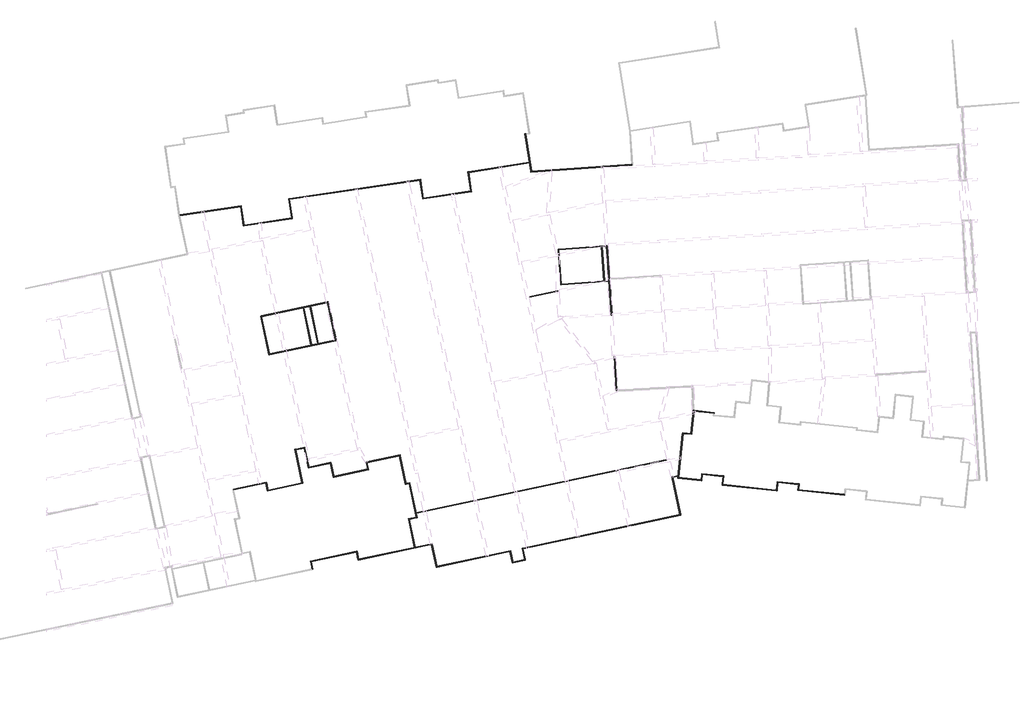
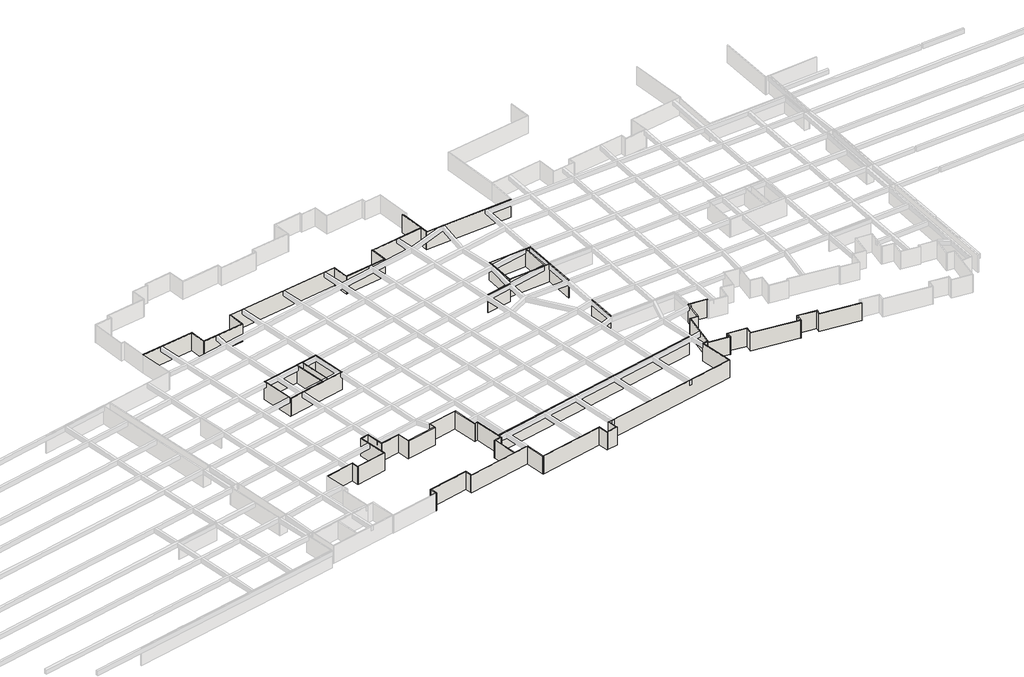
# One storey, part 3 of 14: 67 walls.
"""IFC4 building model written with IfcOpenShell, lengths in millimetres."""

from ifc_helpers import new_model, si_unit, origin, origin_with_axes, place, context, project, spatial, polyline, outline, extrude, faceted_brep, element, save

model = new_model("IFC4")

# Units and contexts
model_context = context("Model", 3, world=origin())
ifc_project = project(units=[si_unit("LENGTHUNIT", "METRE", prefix="MILLI")], contexts=[model_context])

# Site, building, storey
site = spatial("IfcSite", under=ifc_project)
building = spatial("IfcBuilding", under=site)
storey = spatial("IfcBuildingStorey", under=building, Name="户型图", Elevation=0.0)

# Walls
placement = place(None, origin())
element("IfcWall", 1, ObjectType="所有墙体", at=placement, inside=storey, context=model_context, shape_type="Brep", body=[
    faceted_brep([(-251184.7932427, -180181.6677158, 0.0), (-246225.4514721, -179127.5270809, 0.0), (-246108.07376, -179102.577678, 0.0), (-246108.07376, -179102.577678, 3300.0), (-246225.4514721, -179127.5270809, 3300.0), (-251184.7932427, -180181.6677158, 3300.0), (-251209.7426456, -180064.2900037, 0.0), (-251209.7426456, -180064.2900037, 3300.0), (-246133.0231629, -178985.1999659, 3300.0), (-246133.0231629, -178985.1999659, 0.0)], [[[0, 1, 2, 3, 4, 5]], [[6, 7, 8, 9]], [[2, 1, 0, 6, 9]], [[5, 4, 3, 8, 7]], [[0, 5, 7, 6]], [[3, 2, 9, 8]]]),
])
element("IfcWall", 2, ObjectType="所有墙体", at=placement, inside=storey, context=model_context, shape_type="Brep", body=[
    faceted_brep([(-246225.4514721, -179127.5270809, 0.0), (-245969.2063711, -180333.0654988, 0.0), (-245969.2063711, -180333.0654988, 3300.0), (-246225.4514721, -179127.5270809, 3300.0), (-246108.07376, -179102.577678, 0.0), (-246108.07376, -179102.577678, 3300.0), (-245876.7780619, -180190.7383838, 3300.0), (-245851.828659, -180308.1160959, 3300.0), (-245851.828659, -180308.1160959, 0.0), (-245876.7780619, -180190.7383838, 0.0)], [[[0, 1, 2, 3]], [[4, 5, 6, 7, 8, 9]], [[1, 0, 4, 9, 8]], [[3, 2, 7, 6, 5]], [[0, 3, 5, 4]], [[2, 1, 8, 7]]]),
])
element("IfcWall", 3, ObjectType="所有墙体", at=placement, inside=storey, context=model_context, shape_type="Brep", body=[
    faceted_brep([(-245851.828659, -180308.1160959, 0.0), (-240528.356814, -179176.5772244, 0.0), (-240528.356814, -179176.5772244, 3300.0), (-245851.828659, -180308.1160959, 3300.0), (-245876.7780619, -180190.7383838, 0.0), (-245876.7780619, -180190.7383838, 3300.0), (-240670.683929, -179084.1489152, 3300.0), (-240553.3062169, -179059.1995123, 3300.0), (-240553.3062169, -179059.1995123, 0.0), (-240670.683929, -179084.1489152, 0.0)], [[[0, 1, 2, 3]], [[4, 5, 6, 7, 8, 9]], [[1, 0, 4, 9, 8]], [[3, 2, 7, 6, 5]], [[0, 3, 5, 4]], [[2, 1, 8, 7]]]),
])
element("IfcWall", 4, ObjectType="所有墙体", at=placement, inside=storey, context=model_context, shape_type="Brep", body=[
    faceted_brep([(-240553.3062169, -179059.1995123, 0.0), (-241623.2362036, -174025.5746821, 0.0), (-241648.1856065, -173908.19697, 0.0), (-241648.1856065, -173908.19697, 3300.0), (-241623.2362036, -174025.5746821, 3300.0), (-240553.3062169, -179059.1995123, 3300.0), (-240670.683929, -179084.1489152, 0.0), (-240670.683929, -179084.1489152, 3300.0), (-241765.5633186, -173933.1463729, 3300.0), (-241765.5633186, -173933.1463729, 0.0)], [[[0, 1, 2, 3, 4, 5]], [[6, 7, 8, 9]], [[2, 1, 0, 6, 9]], [[5, 4, 3, 8, 7]], [[0, 5, 7, 6]], [[3, 2, 9, 8]]]),
])
element("IfcWall", 5, ObjectType="所有墙体", at=placement, inside=storey, context=model_context, shape_type="Brep", body=[
    faceted_brep([(-241623.2362036, -174025.5746821, 0.0), (-240338.9777317, -173752.597117, 0.0), (-240221.6000196, -173727.6477141, 0.0), (-240221.6000196, -173727.6477141, 3300.0), (-240338.9777317, -173752.597117, 3300.0), (-241623.2362036, -174025.5746821, 3300.0), (-241648.1856065, -173908.19697, 0.0), (-241648.1856065, -173908.19697, 3300.0), (-240246.5494225, -173610.270002, 3300.0), (-240246.5494225, -173610.270002, 0.0)], [[[0, 1, 2, 3, 4, 5]], [[6, 7, 8, 9]], [[2, 1, 0, 6, 9]], [[5, 4, 3, 8, 7]], [[0, 5, 7, 6]], [[3, 2, 9, 8]]]),
])
element("IfcWall", 6, ObjectType="所有墙体", at=placement, inside=storey, context=model_context, shape_type="Brep", body=[
    faceted_brep([(-240338.9777317, -173752.597117, 0.0), (-239692.5763399, -176793.6765678, 0.0), (-239692.5763399, -176793.6765678, 3300.0), (-240338.9777317, -173752.597117, 3300.0), (-240221.6000196, -173727.6477141, 0.0), (-240221.6000196, -173727.6477141, 3300.0), (-239600.1480307, -176651.3494528, 3300.0), (-239575.1986278, -176768.7271649, 3300.0), (-239575.1986278, -176768.7271649, 0.0), (-239600.1480307, -176651.3494528, 0.0)], [[[0, 1, 2, 3]], [[4, 5, 6, 7, 8, 9]], [[1, 0, 4, 9, 8]], [[3, 2, 7, 6, 5]], [[0, 3, 5, 4]], [[2, 1, 8, 7]]]),
])
element("IfcWall", 7, ObjectType="所有墙体", at=placement, inside=storey, context=model_context, shape_type="Brep", body=[
    faceted_brep([(-239575.1986278, -176768.7271649, 0.0), (-236288.0048587, -176070.0125598, 0.0), (-236170.6271466, -176045.0631569, 0.0), (-236170.6271466, -176045.0631569, 3300.0), (-236288.0048587, -176070.0125598, 3300.0), (-239575.1986278, -176768.7271649, 3300.0), (-239600.1480307, -176651.3494528, 0.0), (-239600.1480307, -176651.3494528, 3300.0), (-236195.5765495, -175927.6854448, 3300.0), (-236195.5765495, -175927.6854448, 0.0)], [[[0, 1, 2, 3, 4, 5]], [[6, 7, 8, 9]], [[2, 1, 0, 6, 9]], [[5, 4, 3, 8, 7]], [[0, 5, 7, 6]], [[3, 2, 9, 8]]]),
])
element("IfcWall", 8, ObjectType="所有墙体", at=placement, inside=storey, context=model_context, shape_type="Brep", body=[
    faceted_brep([(-236288.0048587, -176070.0125598, 0.0), (-235830.5991389, -178221.9372814, 0.0), (-235830.5991389, -178221.9372814, 3300.0), (-236288.0048587, -176070.0125598, 3300.0), (-236170.6271466, -176045.0631569, 0.0), (-236170.6271466, -176045.0631569, 3300.0), (-235738.1708297, -178079.6101664, 3300.0), (-235713.2214268, -178196.9878785, 3300.0), (-235713.2214268, -178196.9878785, 0.0), (-235738.1708297, -178079.6101664, 0.0)], [[[0, 1, 2, 3]], [[4, 5, 6, 7, 8, 9]], [[1, 0, 4, 9, 8]], [[3, 2, 7, 6, 5]], [[0, 3, 5, 4]], [[2, 1, 8, 7]]]),
])
element("IfcWall", 9, ObjectType="所有墙体", at=placement, inside=storey, context=model_context, shape_type="Brep", body=[
    faceted_brep([(-235713.2214268, -178196.9878785, 0.0), (-230395.6661839, -177066.7066196, 0.0), (-230395.6661839, -177066.7066196, 3300.0), (-235713.2214268, -178196.9878785, 3300.0), (-235738.1708297, -178079.6101664, 0.0), (-235738.1708297, -178079.6101664, 3300.0), (-230537.9932989, -176974.2783104, 3300.0), (-230420.6155868, -176949.3289075, 3300.0), (-230420.6155868, -176949.3289075, 0.0), (-230537.9932989, -176974.2783104, 0.0)], [[[0, 1, 2, 3]], [[4, 5, 6, 7, 8, 9]], [[1, 0, 4, 9, 8]], [[3, 2, 7, 6, 5]], [[0, 3, 5, 4]], [[2, 1, 8, 7]]]),
])
element("IfcWall", 10, ObjectType="所有墙体", at=placement, inside=storey, context=model_context, shape_type="Brep", body=[
    faceted_brep([(-230420.6155868, -176949.3289075, 0.0), (-230627.4632891, -175976.186979, 0.0), (-230652.412692, -175858.809267, 0.0), (-230652.412692, -175858.809267, 3300.0), (-230627.4632891, -175976.186979, 3300.0), (-230420.6155868, -176949.3289075, 3300.0), (-230537.9932989, -176974.2783104, 0.0), (-230537.9932989, -176974.2783104, 3300.0), (-230769.7904041, -175883.7586699, 3300.0), (-230769.7904041, -175883.7586699, 0.0)], [[[0, 1, 2, 3, 4, 5]], [[6, 7, 8, 9]], [[2, 1, 0, 6, 9]], [[5, 4, 3, 8, 7]], [[0, 5, 7, 6]], [[3, 2, 9, 8]]]),
])
element("IfcWall", 11, ObjectType="所有墙体", at=placement, inside=storey, context=model_context, shape_type="Brep", body=[
    faceted_brep([(-230627.4632891, -175976.186979, 0.0), (-225651.5563884, -174918.525317, 0.0), (-225534.1786764, -174893.5759141, 0.0), (-225534.1786764, -174893.5759141, 3300.0), (-225651.5563884, -174918.525317, 3300.0), (-230627.4632891, -175976.186979, 3300.0), (-230652.412692, -175858.809267, 0.0), (-230652.412692, -175858.809267, 3300.0), (-225559.1280793, -174776.1982021, 3300.0), (-225559.1280793, -174776.1982021, 0.0)], [[[0, 1, 2, 3, 4, 5]], [[6, 7, 8, 9]], [[2, 1, 0, 6, 9]], [[5, 4, 3, 8, 7]], [[0, 5, 7, 6]], [[3, 2, 9, 8]]]),
])
element("IfcWall", 12, ObjectType="所有墙体", at=placement, inside=storey, context=model_context, shape_type="Brep", body=[
    faceted_brep([(-225651.5563884, -174918.525317, 0.0), (-224715.2696958, -179323.4078824, 0.0), (-224715.2696958, -179323.4078824, 3300.0), (-225651.5563884, -174918.525317, 3300.0), (-225534.1786764, -174893.5759141, 0.0), (-225534.1786764, -174893.5759141, 3300.0), (-224622.8413866, -179181.0807674, 3300.0), (-224597.8919837, -179298.4584795, 3300.0), (-224597.8919837, -179298.4584795, 0.0), (-224622.8413866, -179181.0807674, 0.0)], [[[0, 1, 2, 3]], [[4, 5, 6, 7, 8, 9]], [[1, 0, 4, 9, 8]], [[3, 2, 7, 6, 5]], [[0, 3, 5, 4]], [[2, 1, 8, 7]]]),
])
element("IfcWall", 13, ObjectType="所有墙体", at=placement, inside=storey, context=model_context, shape_type="Brep", body=[
    faceted_brep([(-224597.8919837, -179298.4584795, 0.0), (-224155.9078939, -179204.5118611, 0.0), (-224038.5301818, -179179.5624582, 0.0), (-224038.5301818, -179179.5624582, 3300.0), (-224155.9078939, -179204.5118611, 3300.0), (-224597.8919837, -179298.4584795, 3300.0), (-224622.8413866, -179181.0807674, 0.0), (-224622.8413866, -179181.0807674, 3300.0), (-224063.4795847, -179062.1847461, 3300.0), (-224063.4795847, -179062.1847461, 0.0)], [[[0, 1, 2, 3, 4, 5]], [[6, 7, 8, 9]], [[2, 1, 0, 6, 9]], [[5, 4, 3, 8, 7]], [[0, 5, 7, 6]], [[3, 2, 9, 8]]]),
])
element("IfcWall", 14, ObjectType="所有墙体", at=placement, inside=storey, context=model_context, shape_type="Brep", body=[
    faceted_brep([(-224155.9078939, -179204.5118611, 0.0), (-223057.3689575, -184372.7312177, 0.0), (-223032.4195546, -184490.1089298, 0.0), (-223032.4195546, -184490.1089298, 3300.0), (-223057.3689575, -184372.7312177, 3300.0), (-224155.9078939, -179204.5118611, 3300.0), (-224038.5301818, -179179.5624582, 0.0), (-224038.5301818, -179179.5624582, 3300.0), (-223083.6040764, -183672.1365659, 3300.0), (-223058.6546735, -183789.5142779, 3300.0), (-222915.0418425, -184465.1595269, 3300.0), (-222915.0418425, -184465.1595269, 0.0), (-223058.6546735, -183789.5142779, 0.0), (-223083.6040764, -183672.1365659, 0.0)], [[[0, 1, 2, 3, 4, 5]], [[6, 7, 8, 9, 10, 11, 12, 13]], [[2, 1, 0, 6, 13, 12, 11]], [[5, 4, 3, 10, 9, 8, 7]], [[0, 5, 7, 6]], [[3, 2, 11, 10]]]),
])
element("IfcWall", 15, ObjectType="所有墙体", at=placement, inside=storey, context=model_context, shape_type="Brep", body=[
    faceted_brep([(-223057.3689575, -184372.7312177, 0.0), (-224264.2132514, -184629.2538913, 0.0), (-224264.2132514, -184629.2538913, 3300.0), (-223057.3689575, -184372.7312177, 3300.0), (-223032.4195546, -184490.1089298, 0.0), (-223032.4195546, -184490.1089298, 3300.0), (-224121.8861364, -184721.6822004, 3300.0), (-224239.2638485, -184746.6316033, 3300.0), (-224239.2638485, -184746.6316033, 0.0), (-224121.8861364, -184721.6822004, 0.0)], [[[0, 1, 2, 3]], [[4, 5, 6, 7, 8, 9]], [[1, 0, 4, 9, 8]], [[3, 2, 7, 6, 5]], [[0, 3, 5, 4]], [[2, 1, 8, 7]]]),
])
element("IfcWall", 16, ObjectType="所有墙体", at=placement, inside=storey, context=model_context, shape_type="SweptSolid", body=[
    extrude(outline(polyline([(-223330.1960749, -189023.4592223), (-224239.2638485, -184746.6316033), (-224121.8861364, -184721.6822004), (-223212.8183628, -188998.5098194), (-223330.1960749, -189023.4592223)])), origin_with_axes(), (0.0, 0.0, 1.0), 3300.0),
])
element("IfcWall", 17, ObjectType="所有墙体", at=placement, inside=storey, context=model_context, shape_type="Brep", body=[
    faceted_brep([(-220629.7896191, -188449.4701109, 0.0), (-223212.8183628, -188998.5098194, 0.0), (-223330.1960749, -189023.4592223, 0.0), (-231918.3320094, -190848.9238676, 0.0), (-232035.7097215, -190873.8732705, 0.0), (-232035.7097215, -190873.8732705, 3300.0), (-231918.3320094, -190848.9238676, 3300.0), (-223330.1960749, -189023.4592223, 3300.0), (-223212.8183628, -188998.5098194, 3300.0), (-220629.7896191, -188449.4701109, 3300.0), (-220604.8402162, -188566.847823, 0.0), (-220604.8402162, -188566.847823, 3300.0), (-220722.2179283, -188591.7972259, 3300.0), (-232010.7603186, -190991.2509826, 3300.0), (-232010.7603186, -190991.2509826, 0.0), (-220722.2179283, -188591.7972259, 0.0)], [[[0, 1, 2, 3, 4, 5, 6, 7, 8, 9]], [[10, 11, 12, 13, 14, 15]], [[4, 3, 2, 1, 0, 10, 15, 14]], [[9, 8, 7, 6, 5, 13, 12, 11]], [[5, 4, 14, 13]], [[0, 9, 11, 10]]]),
])
element("IfcWall", 18, ObjectType="所有墙体", at=placement, inside=storey, context=model_context, shape_type="Brep", body=[
    faceted_brep([(-231918.3320094, -190848.9238676, 0.0), (-232179.3992418, -189620.6991054, 0.0), (-232179.3992418, -189620.6991054, 3300.0), (-231918.3320094, -190848.9238676, 3300.0), (-232035.7097215, -190873.8732705, 0.0), (-232035.7097215, -190873.8732705, 3300.0), (-232271.827551, -189763.0262204, 3300.0), (-232296.7769539, -189645.6485083, 3300.0), (-232296.7769539, -189645.6485083, 0.0), (-232271.827551, -189763.0262204, 0.0)], [[[0, 1, 2, 3]], [[4, 5, 6, 7, 8, 9]], [[1, 0, 4, 9, 8]], [[3, 2, 7, 6, 5]], [[0, 3, 5, 4]], [[2, 1, 8, 7]]]),
])
element("IfcWall", 19, ObjectType="所有墙体", at=placement, inside=storey, context=model_context, shape_type="Brep", body=[
    faceted_brep([(-232296.7769539, -189645.6485083, 0.0), (-239359.5403512, -191146.885212, 0.0), (-239359.5403512, -191146.885212, 3300.0), (-232296.7769539, -189645.6485083, 3300.0), (-232271.827551, -189763.0262204, 0.0), (-232271.827551, -189763.0262204, 3300.0), (-239217.2132362, -191239.3135211, 3300.0), (-239334.5909483, -191264.262924, 3300.0), (-239334.5909483, -191264.262924, 0.0), (-239217.2132362, -191239.3135211, 0.0)], [[[0, 1, 2, 3]], [[4, 5, 6, 7, 8, 9]], [[1, 0, 4, 9, 8]], [[3, 2, 7, 6, 5]], [[0, 3, 5, 4]], [[2, 1, 8, 7]]]),
])
element("IfcWall", 20, ObjectType="所有墙体", at=placement, inside=storey, context=model_context, shape_type="Brep", body=[
    faceted_brep([(-239334.5909483, -191264.262924, 0.0), (-239110.0463222, -192320.6623328, 0.0), (-239085.0969193, -192438.0400449, 0.0), (-239085.0969193, -192438.0400449, 3300.0), (-239110.0463222, -192320.6623328, 3300.0), (-239334.5909483, -191264.262924, 3300.0), (-239217.2132362, -191239.3135211, 0.0), (-239217.2132362, -191239.3135211, 3300.0), (-238967.7192072, -192413.090642, 3300.0), (-238967.7192072, -192413.090642, 0.0)], [[[0, 1, 2, 3, 4, 5]], [[6, 7, 8, 9]], [[2, 1, 0, 6, 9]], [[5, 4, 3, 8, 7]], [[0, 5, 7, 6]], [[3, 2, 9, 8]]]),
])
element("IfcWall", 21, ObjectType="所有墙体", at=placement, inside=storey, context=model_context, shape_type="Brep", body=[
    faceted_brep([(-182065.556888, -171503.9612716, 0.0), (-181945.9953144, -171514.4215539, 0.0), (-180665.2470066, -171626.4725117, 0.0), (-180665.2470066, -171626.4725117, 3300.0), (-181945.9953144, -171514.4215539, 3300.0), (-182065.556888, -171503.9612716, 3300.0), (-182053.0115616, -171384.6004649, 0.0), (-182053.0115616, -171384.6004649, 3300.0), (-180772.2632539, -171496.6514227, 3300.0), (-180652.7016803, -171507.111705, 3300.0), (-180652.7016803, -171507.111705, 0.0), (-180772.2632539, -171496.6514227, 0.0)], [[[0, 1, 2, 3, 4, 5]], [[6, 7, 8, 9, 10, 11]], [[2, 1, 0, 6, 11, 10]], [[5, 4, 3, 9, 8, 7]], [[3, 2, 10, 9]], [[0, 5, 7, 6]]]),
])
element("IfcWall", 22, ObjectType="所有墙体", at=placement, inside=storey, context=model_context, shape_type="Brep", body=[
    faceted_brep([(-180652.7016803, -171507.111705, 0.0), (-180289.0530565, -168047.2261654, 0.0), (-180276.5096409, -167927.8835379, 0.0), (-180276.5096409, -167927.8835379, 3300.0), (-180289.0530565, -168047.2261654, 3300.0), (-180652.7016803, -171507.111705, 3300.0), (-180772.2632539, -171496.6514227, 0.0), (-180772.2632539, -171496.6514227, 3300.0), (-180402.6175703, -167979.7076703, 3300.0), (-180395.8522684, -167915.3401223, 3300.0), (-180395.8522684, -167915.3401223, 0.0), (-180402.6175703, -167979.7076703, 0.0), (-180285.2168381, -167926.9683746, 0.0), (-180285.2168381, -167926.9683746, 3300.0)], [[[0, 1, 2, 3, 4, 5]], [[6, 7, 8, 9, 10, 11]], [[2, 1, 0, 6, 11, 10, 12]], [[5, 4, 3, 13, 9, 8, 7]], [[0, 5, 7, 6]], [[3, 2, 12, 10, 9, 13]]]),
])
element("IfcWall", 23, ObjectType="所有墙体", at=placement, inside=storey, context=model_context, shape_type="Brep", body=[
    faceted_brep([(-180289.0530565, -168047.2261654, 0.0), (-177282.9502682, -168363.1803001, 0.0), (-177163.6076407, -168375.7237157, 0.0), (-177163.6076407, -168375.7237157, 3300.0), (-177282.9502682, -168363.1803001, 3300.0), (-180289.0530565, -168047.2261654, 3300.0), (-180276.5096409, -167927.8835379, 0.0), (-180276.5096409, -167927.8835379, 3300.0), (-177151.0642251, -168256.3810882, 3300.0), (-177151.0642251, -168256.3810882, 0.0)], [[[0, 1, 2, 3, 4, 5]], [[6, 7, 8, 9]], [[2, 1, 0, 6, 9]], [[5, 4, 3, 8, 7]], [[0, 5, 7, 6]], [[3, 2, 9, 8]]]),
])
element("IfcWall", 24, ObjectType="所有墙体", at=placement, inside=storey, context=model_context, shape_type="Brep", body=[
    faceted_brep([(-157110.1034337, -180872.9468522, 0.0), (-164149.4886008, -180133.0776575, 0.0), (-164268.8312282, -180120.5342419, 0.0), (-164268.8312282, -180120.5342419, 3300.0), (-164149.4886008, -180133.0776575, 3300.0), (-157110.1034337, -180872.9468522, 3300.0), (-157122.6468493, -180992.2894796, 0.0), (-157122.6468493, -180992.2894796, 3300.0), (-164281.3746438, -180239.8768693, 3300.0), (-164281.3746438, -180239.8768693, 0.0)], [[[0, 1, 2, 3, 4, 5]], [[6, 7, 8, 9]], [[2, 1, 0, 6, 9]], [[5, 4, 3, 8, 7]], [[0, 5, 7, 6]], [[3, 2, 9, 8]]]),
])
element("IfcWall", 25, ObjectType="所有墙体", at=placement, inside=storey, context=model_context, shape_type="Brep", body=[
    faceted_brep([(-164149.4886008, -180133.0776575, 0.0), (-164056.3781259, -179247.1906647, 0.0), (-164056.3781259, -179247.1906647, 3300.0), (-164149.4886008, -180133.0776575, 3300.0), (-164268.8312282, -180120.5342419, 0.0), (-164268.8312282, -180120.5342419, 3300.0), (-164188.2641689, -179353.9898766, 3300.0), (-164175.7207533, -179234.6472492, 3300.0), (-164175.7207533, -179234.6472492, 0.0), (-164188.2641689, -179353.9898766, 0.0)], [[[0, 1, 2, 3]], [[4, 5, 6, 7, 8, 9]], [[1, 0, 4, 9, 8]], [[3, 2, 7, 6, 5]], [[0, 3, 5, 4]], [[2, 1, 8, 7]]]),
])
element("IfcWall", 26, ObjectType="所有墙体", at=placement, inside=storey, context=model_context, shape_type="Brep", body=[
    faceted_brep([(-164175.7207533, -179234.6472492, 0.0), (-167459.4955166, -178889.5086139, 0.0), (-167459.4955166, -178889.5086139, 3300.0), (-164175.7207533, -179234.6472492, 3300.0), (-164188.2641689, -179353.9898766, 0.0), (-164188.2641689, -179353.9898766, 3300.0), (-167352.6963048, -179021.3946569, 3300.0), (-167472.0389322, -179008.8512413, 3300.0), (-167472.0389322, -179008.8512413, 0.0), (-167352.6963048, -179021.3946569, 0.0)], [[[0, 1, 2, 3]], [[4, 5, 6, 7, 8, 9]], [[1, 0, 4, 9, 8]], [[3, 2, 7, 6, 5]], [[0, 3, 5, 4]], [[2, 1, 8, 7]]]),
])
element("IfcWall", 27, ObjectType="所有墙体", at=placement, inside=storey, context=model_context, shape_type="Brep", body=[
    faceted_brep([(-167472.0389322, -179008.8512413, 0.0), (-167597.4730882, -180202.2775158, 0.0), (-167610.0165037, -180321.6201432, 0.0), (-167610.0165037, -180321.6201432, 3300.0), (-167597.4730882, -180202.2775158, 3300.0), (-167472.0389322, -179008.8512413, 3300.0), (-167352.6963048, -179021.3946569, 0.0), (-167352.6963048, -179021.3946569, 3300.0), (-167490.6738763, -180334.1635588, 3300.0), (-167490.6738763, -180334.1635588, 0.0)], [[[0, 1, 2, 3, 4, 5]], [[6, 7, 8, 9]], [[2, 1, 0, 6, 9]], [[5, 4, 3, 8, 7]], [[0, 5, 7, 6]], [[3, 2, 9, 8]]]),
])
element("IfcWall", 28, ObjectType="所有墙体", at=placement, inside=storey, context=model_context, shape_type="Brep", body=[
    faceted_brep([(-167597.4730882, -180202.2775158, 0.0), (-175829.3978828, -179337.0673554, 0.0), (-175948.7405103, -179324.5239399, 0.0), (-175948.7405103, -179324.5239399, 3300.0), (-175829.3978828, -179337.0673554, 3300.0), (-167597.4730882, -180202.2775158, 3300.0), (-167610.0165037, -180321.6201432, 0.0), (-167610.0165037, -180321.6201432, 3300.0), (-175961.2839258, -179443.8665673, 3300.0), (-175961.2839258, -179443.8665673, 0.0)], [[[0, 1, 2, 3, 4, 5]], [[6, 7, 8, 9]], [[2, 1, 0, 6, 9]], [[5, 4, 3, 8, 7]], [[0, 5, 7, 6]], [[3, 2, 9, 8]]]),
])
element("IfcWall", 29, ObjectType="所有墙体", at=placement, inside=storey, context=model_context, shape_type="Brep", body=[
    faceted_brep([(-175829.3978828, -179337.0673554, 0.0), (-175691.4203113, -178024.2984536, 0.0), (-175691.4203113, -178024.2984536, 3300.0), (-175829.3978828, -179337.0673554, 3300.0), (-175948.7405103, -179324.5239399, 0.0), (-175948.7405103, -179324.5239399, 3300.0), (-175823.3063543, -178131.0976654, 3300.0), (-175810.7629387, -178011.755038, 3300.0), (-175810.7629387, -178011.755038, 0.0), (-175823.3063543, -178131.0976654, 0.0)], [[[0, 1, 2, 3]], [[4, 5, 6, 7, 8, 9]], [[1, 0, 4, 9, 8]], [[3, 2, 7, 6, 5]], [[0, 3, 5, 4]], [[2, 1, 8, 7]]]),
])
element("IfcWall", 30, ObjectType="所有墙体", at=placement, inside=storey, context=model_context, shape_type="Brep", body=[
    faceted_brep([(-175810.7629387, -178011.755038, 0.0), (-179092.6851935, -177666.8111092, 0.0), (-179092.6851935, -177666.8111092, 3300.0), (-175810.7629387, -178011.755038, 3300.0), (-175823.3063543, -178131.0976654, 0.0), (-175823.3063543, -178131.0976654, 3300.0), (-178985.8859816, -177798.6971522, 3300.0), (-179105.228609, -177786.1537366, 3300.0), (-179105.228609, -177786.1537366, 0.0), (-178985.8859816, -177798.6971522, 0.0)], [[[0, 1, 2, 3]], [[4, 5, 6, 7, 8, 9]], [[1, 0, 4, 9, 8]], [[3, 2, 7, 6, 5]], [[0, 3, 5, 4]], [[2, 1, 8, 7]]]),
])
element("IfcWall", 31, ObjectType="所有墙体", at=placement, inside=storey, context=model_context, shape_type="Brep", body=[
    faceted_brep([(-179105.228609, -177786.1537366, 0.0), (-179192.313451, -178614.7106614, 0.0), (-179204.8568666, -178734.0532889, 0.0), (-179204.8568666, -178734.0532889, 3300.0), (-179192.313451, -178614.7106614, 3300.0), (-179105.228609, -177786.1537366, 3300.0), (-178985.8859816, -177798.6971522, 0.0), (-178985.8859816, -177798.6971522, 3300.0), (-179085.5142391, -178746.5967045, 3300.0), (-179085.5142391, -178746.5967045, 0.0)], [[[0, 1, 2, 3, 4, 5]], [[6, 7, 8, 9]], [[2, 1, 0, 6, 9]], [[5, 4, 3, 8, 7]], [[0, 5, 7, 6]], [[3, 2, 9, 8]]]),
])
element("IfcWall", 32, ObjectType="所有墙体", at=placement, inside=storey, context=model_context, shape_type="Brep", body=[
    faceted_brep([(-179192.313451, -178614.7106614, 0.0), (-182654.0245934, -178250.8701591, 0.0), (-182773.3672209, -178238.3267435, 0.0), (-182773.3672209, -178238.3267435, 3300.0), (-182654.0245934, -178250.8701591, 3300.0), (-179192.313451, -178614.7106614, 3300.0), (-179204.8568666, -178734.0532889, 0.0), (-179204.8568666, -178734.0532889, 3300.0), (-182785.9106365, -178357.669371, 3300.0), (-182785.9106365, -178357.669371, 0.0)], [[[0, 1, 2, 3, 4, 5]], [[6, 7, 8, 9]], [[2, 1, 0, 6, 9]], [[5, 4, 3, 8, 7]], [[0, 5, 7, 6]], [[3, 2, 9, 8]]]),
])
element("IfcWall", 33, ObjectType="所有墙体", at=placement, inside=storey, context=model_context, shape_type="Brep", body=[
    faceted_brep([(-182654.0245934, -178250.8701591, 0.0), (-181945.9953144, -171514.4215539, 0.0), (-181945.9953144, -171514.4215539, 3300.0), (-182654.0245934, -178250.8701591, 3300.0), (-182773.3672209, -178238.3267435, 0.0), (-182773.3672209, -178238.3267435, 3300.0), (-182757.9194792, -178091.3512993, 3300.0), (-182744.7305516, -177965.8670348, 3300.0), (-182065.556888, -171503.9612716, 3300.0), (-182065.556888, -171503.9612716, 0.0), (-182744.7305516, -177965.8670348, 0.0), (-182757.9194792, -178091.3512993, 0.0)], [[[0, 1, 2, 3]], [[4, 5, 6, 7, 8, 9, 10, 11]], [[1, 0, 4, 11, 10, 9]], [[3, 2, 8, 7, 6, 5]], [[2, 1, 9, 8]], [[0, 3, 5, 4]]]),
])
element("IfcWall", 34, ObjectType="所有墙体", at=placement, inside=storey, context=model_context, shape_type="Brep", body=[
    faceted_brep([(-205290.7605884, -131109.081479, 0.0), (-206189.3856367, -125435.3862189, 0.0), (-206208.1577725, -125316.863618, 0.0), (-206208.1577725, -125316.863618, 3300.0), (-206189.3856367, -125435.3862189, 3300.0), (-205290.7605884, -131109.081479, 3300.0), (-205410.9255383, -131117.4842309, 0.0), (-205410.9255383, -131117.4842309, 3300.0), (-205617.1977326, -129815.132852, 3300.0), (-205635.9698684, -129696.6102511, 3300.0), (-206326.6803734, -125335.6357538, 3300.0), (-206326.6803734, -125335.6357538, 0.0), (-205635.9698684, -129696.6102511, 0.0), (-205617.1977326, -129815.132852, 0.0)], [[[0, 1, 2, 3, 4, 5]], [[6, 7, 8, 9, 10, 11, 12, 13]], [[2, 1, 0, 6, 13, 12, 11]], [[5, 4, 3, 10, 9, 8, 7]], [[3, 2, 11, 10]], [[0, 5, 7, 6]]]),
])
element("IfcWall", 35, ObjectType="所有墙体", at=placement, inside=storey, context=model_context, shape_type="Brep", body=[
    faceted_brep([(-259497.8296146, -137947.3843831, 0.0), (-259493.9278671, -137946.8113411, 0.0), (-250107.6507443, -136568.2671346, 0.0), (-249988.9243897, -136550.8300265, 0.0), (-249988.9243897, -136550.8300265, 3300.0), (-250107.6507443, -136568.2671346, 3300.0), (-259493.9278671, -137946.8113411, 3300.0), (-259497.8296146, -137947.3843831, 3300.0), (-259515.2667226, -137828.6580286, 0.0), (-259515.2667226, -137828.6580286, 3300.0), (-250006.3614978, -136432.103672, 3300.0), (-250006.3614978, -136432.103672, 0.0)], [[[0, 1, 2, 3, 4, 5, 6, 7]], [[8, 9, 10, 11]], [[3, 2, 1, 0, 8, 11]], [[7, 6, 5, 4, 10, 9]], [[0, 7, 9, 8]], [[4, 3, 11, 10]]]),
])
element("IfcWall", 36, ObjectType="所有墙体", at=placement, inside=storey, context=model_context, shape_type="Brep", body=[
    faceted_brep([(-250107.6507443, -136568.2671346, 0.0), (-249675.1126294, -139513.3468741, 0.0), (-249675.1126294, -139513.3468741, 3300.0), (-250107.6507443, -136568.2671346, 3300.0), (-249988.9243897, -136550.8300265, 0.0), (-249988.9243897, -136550.8300265, 3300.0), (-249573.8233829, -139377.1834115, 3300.0), (-249556.3862748, -139495.9097661, 3300.0), (-249556.3862748, -139495.9097661, 0.0), (-249573.8233829, -139377.1834115, 0.0)], [[[0, 1, 2, 3]], [[4, 5, 6, 7, 8, 9]], [[1, 0, 4, 9, 8]], [[3, 2, 7, 6, 5]], [[0, 3, 5, 4]], [[2, 1, 8, 7]]]),
])
element("IfcWall", 37, ObjectType="所有墙体", at=placement, inside=storey, context=model_context, shape_type="Brep", body=[
    faceted_brep([(-249556.3862748, -139495.9097661, 0.0), (-242128.8165149, -138405.0370881, 0.0), (-242128.8165149, -138405.0370881, 3300.0), (-249556.3862748, -139495.9097661, 3300.0), (-249573.8233829, -139377.1834115, 0.0), (-249573.8233829, -139377.1834115, 3300.0), (-242264.9799775, -138303.7478416, 3300.0), (-242146.253623, -138286.3107336, 3300.0), (-242146.253623, -138286.3107336, 0.0), (-242264.9799775, -138303.7478416, 0.0)], [[[0, 1, 2, 3]], [[4, 5, 6, 7, 8, 9]], [[1, 0, 4, 9, 8]], [[3, 2, 7, 6, 5]], [[0, 3, 5, 4]], [[2, 1, 8, 7]]]),
])
element("IfcWall", 38, ObjectType="所有墙体", at=placement, inside=storey, context=model_context, shape_type="Brep", body=[
    faceted_brep([(-242146.253623, -138286.3107336, 0.0), (-242564.7442158, -135436.8782245, 0.0), (-242582.1813238, -135318.15187, 0.0), (-242582.1813238, -135318.15187, 3300.0), (-242564.7442158, -135436.8782245, 3300.0), (-242146.253623, -138286.3107336, 3300.0), (-242264.9799775, -138303.7478416, 0.0), (-242264.9799775, -138303.7478416, 3300.0), (-242700.9076783, -135335.588978, 3300.0), (-242700.9076783, -135335.588978, 0.0)], [[[0, 1, 2, 3, 4, 5]], [[6, 7, 8, 9]], [[2, 1, 0, 6, 9]], [[5, 4, 3, 8, 7]], [[0, 5, 7, 6]], [[3, 2, 9, 8]]]),
])
element("IfcWall", 39, ObjectType="所有墙体", at=placement, inside=storey, context=model_context, shape_type="Brep", body=[
    faceted_brep([(-242564.7442158, -135436.8782245, 0.0), (-222499.9902977, -132490.006967, 0.0), (-222381.2639432, -132472.5698589, 0.0), (-222381.2639432, -132472.5698589, 3300.0), (-222499.9902977, -132490.006967, 3300.0), (-242564.7442158, -135436.8782245, 3300.0), (-242582.1813238, -135318.15187, 0.0), (-242582.1813238, -135318.15187, 3300.0), (-222398.7010512, -132353.8435044, 3300.0), (-222398.7010512, -132353.8435044, 0.0)], [[[0, 1, 2, 3, 4, 5]], [[6, 7, 8, 9]], [[2, 1, 0, 6, 9]], [[5, 4, 3, 8, 7]], [[0, 5, 7, 6]], [[3, 2, 9, 8]]]),
])
element("IfcWall", 40, ObjectType="所有墙体", at=placement, inside=storey, context=model_context, shape_type="Brep", body=[
    faceted_brep([(-222499.9902977, -132490.006967, 0.0), (-222078.5935203, -135359.2272018, 0.0), (-222078.5935203, -135359.2272018, 3300.0), (-222499.9902977, -132490.006967, 3300.0), (-222381.2639432, -132472.5698589, 0.0), (-222381.2639432, -132472.5698589, 3300.0), (-221977.3042738, -135223.0637392, 3300.0), (-221959.8671657, -135341.7900938, 3300.0), (-221959.8671657, -135341.7900938, 0.0), (-221977.3042738, -135223.0637392, 0.0)], [[[0, 1, 2, 3]], [[4, 5, 6, 7, 8, 9]], [[1, 0, 4, 9, 8]], [[3, 2, 7, 6, 5]], [[0, 3, 5, 4]], [[2, 1, 8, 7]]]),
])
element("IfcWall", 41, ObjectType="所有墙体", at=placement, inside=storey, context=model_context, shape_type="Brep", body=[
    faceted_brep([(-221959.8671657, -135341.7900938, 0.0), (-214539.6288625, -134251.9941726, 0.0), (-214539.6288625, -134251.9941726, 3300.0), (-221959.8671657, -135341.7900938, 3300.0), (-221977.3042738, -135223.0637392, 0.0), (-221977.3042738, -135223.0637392, 3300.0), (-214675.7923251, -134150.7049261, 3300.0), (-214557.0659706, -134133.267818, 3300.0), (-214557.0659706, -134133.267818, 0.0), (-214675.7923251, -134150.7049261, 0.0)], [[[0, 1, 2, 3]], [[4, 5, 6, 7, 8, 9]], [[1, 0, 4, 9, 8]], [[3, 2, 7, 6, 5]], [[0, 3, 5, 4]], [[2, 1, 8, 7]]]),
])
element("IfcWall", 42, ObjectType="所有墙体", at=placement, inside=storey, context=model_context, shape_type="Brep", body=[
    faceted_brep([(-214557.0659706, -134133.267818, 0.0), (-214973.6166255, -131297.0440218, 0.0), (-214991.0548378, -131178.3101482, 0.0), (-214991.0548378, -131178.3101482, 3300.0), (-214973.6166255, -131297.0440218, 3300.0), (-214557.0659706, -134133.267818, 3300.0), (-214675.7923251, -134150.7049261, 0.0), (-214675.7923251, -134150.7049261, 3300.0), (-215109.5849448, -131197.0834728, 3300.0), (-215109.5849448, -131197.0834728, 0.0)], [[[0, 1, 2, 3, 4, 5]], [[6, 7, 8, 9]], [[2, 1, 0, 6, 9]], [[5, 4, 3, 8, 7]], [[0, 5, 7, 6]], [[3, 2, 9, 8]]]),
])
element("IfcWall", 43, ObjectType="所有墙体", at=placement, inside=storey, context=model_context, shape_type="SweptSolid", body=[
    extrude(outline(polyline([(-205617.1977326, -129815.132852), (-214973.6166255, -131297.0440218), (-214991.0548378, -131178.3101482), (-205635.9698684, -129696.6102511), (-205617.1977326, -129815.132852)])), origin_with_axes(), (0.0, 0.0, 1.0), 3300.0),
])
element("IfcWall", 44, ObjectType="所有墙体", at=placement, inside=storey, context=model_context, shape_type="Brep", body=[
    faceted_brep([(-220722.2179283, -188591.7972259, 0.0), (-219980.530919, -192081.160262, 0.0), (-219980.530919, -192081.160262, 3300.0), (-220722.2179283, -188591.7972259, 3300.0), (-220604.8402162, -188566.847823, 0.0), (-220604.8402162, -188566.847823, 3300.0), (-219888.1026098, -191938.833147, 3300.0), (-219863.1532069, -192056.2108591, 3300.0), (-219863.1532069, -192056.2108591, 0.0), (-219888.1026098, -191938.833147, 0.0)], [[[0, 1, 2, 3]], [[4, 5, 6, 7, 8, 9]], [[1, 0, 4, 9, 8]], [[3, 2, 7, 6, 5]], [[0, 3, 5, 4]], [[2, 1, 8, 7]]]),
])
element("IfcWall", 45, ObjectType="所有墙体", at=placement, inside=storey, context=model_context, shape_type="Brep", body=[
    faceted_brep([(-219863.1532069, -192056.2108591, 0.0), (-208633.2511205, -189669.2214837, 0.0), (-208515.8734085, -189644.2720808, 0.0), (-208515.8734085, -189644.2720808, 3300.0), (-208633.2511205, -189669.2214837, 3300.0), (-219863.1532069, -192056.2108591, 3300.0), (-219888.1026098, -191938.833147, 0.0), (-219888.1026098, -191938.833147, 3300.0), (-208540.8228113, -189526.8943687, 3300.0), (-208540.8228113, -189526.8943687, 0.0)], [[[0, 1, 2, 3, 4, 5]], [[6, 7, 8, 9]], [[2, 1, 0, 6, 9]], [[5, 4, 3, 8, 7]], [[0, 5, 7, 6]], [[3, 2, 9, 8]]]),
])
element("IfcWall", 46, ObjectType="所有墙体", at=placement, inside=storey, context=model_context, shape_type="Brep", body=[
    faceted_brep([(-208633.2511205, -189669.2214837, 0.0), (-208259.5404842, -191427.3917957, 0.0), (-208259.5404842, -191427.3917957, 3300.0), (-208633.2511205, -189669.2214837, 3300.0), (-208515.8734085, -189644.2720808, 0.0), (-208515.8734085, -189644.2720808, 3300.0), (-208167.112175, -191285.0646807, 3300.0), (-208142.1627721, -191402.4423928, 3300.0), (-208142.1627721, -191402.4423928, 0.0), (-208167.112175, -191285.0646807, 0.0)], [[[0, 1, 2, 3]], [[4, 5, 6, 7, 8, 9]], [[1, 0, 4, 9, 8]], [[3, 2, 7, 6, 5]], [[0, 3, 5, 4]], [[2, 1, 8, 7]]]),
])
element("IfcWall", 47, ObjectType="所有墙体", at=placement, inside=storey, context=model_context, shape_type="Brep", body=[
    faceted_brep([(-208142.1627721, -191402.4423928, 0.0), (-206234.3882604, -190996.9324022, 0.0), (-206234.3882604, -190996.9324022, 3300.0), (-208142.1627721, -191402.4423928, 3300.0), (-208167.112175, -191285.0646807, 0.0), (-208167.112175, -191285.0646807, 3300.0), (-206376.7153754, -190904.504093, 3300.0), (-206259.3376633, -190879.5546901, 3300.0), (-206259.3376633, -190879.5546901, 0.0), (-206376.7153754, -190904.504093, 0.0)], [[[0, 1, 2, 3]], [[4, 5, 6, 7, 8, 9]], [[1, 0, 4, 9, 8]], [[3, 2, 7, 6, 5]], [[0, 3, 5, 4]], [[2, 1, 8, 7]]]),
])
element("IfcWall", 48, ObjectType="所有墙体", at=placement, inside=storey, context=model_context, shape_type="Brep", body=[
    faceted_brep([(-206259.3376633, -190879.5546901, 0.0), (-206608.0988968, -189238.7620902, 0.0), (-206633.0482997, -189121.3843781, 0.0), (-206633.0482997, -189121.3843781, 3300.0), (-206608.0988968, -189238.7620902, 3300.0), (-206259.3376633, -190879.5546901, 3300.0), (-206376.7153754, -190904.504093, 0.0), (-206376.7153754, -190904.504093, 3300.0), (-206750.4260118, -189146.333781, 3300.0), (-206750.4260118, -189146.333781, 0.0)], [[[0, 1, 2, 3, 4, 5]], [[6, 7, 8, 9]], [[2, 1, 0, 6, 9]], [[5, 4, 3, 8, 7]], [[0, 5, 7, 6]], [[3, 2, 9, 8]]]),
])
element("IfcWall", 49, ObjectType="所有墙体", at=placement, inside=storey, context=model_context, shape_type="Brep", body=[
    faceted_brep([(-206608.0988968, -189238.7620902, 0.0), (-182301.5170749, -184072.2386322, 0.0), (-182301.5170749, -184072.2386322, 3300.0), (-206608.0988968, -189238.7620902, 3300.0), (-206633.0482997, -189121.3843781, 0.0), (-206633.0482997, -189121.3843781, 3300.0), (-182443.8441899, -183979.810323, 3300.0), (-182326.4664778, -183954.8609201, 3300.0), (-182326.4664778, -183954.8609201, 0.0), (-182443.8441899, -183979.810323, 0.0)], [[[0, 1, 2, 3]], [[4, 5, 6, 7, 8, 9]], [[1, 0, 4, 9, 8]], [[3, 2, 7, 6, 5]], [[0, 3, 5, 4]], [[2, 1, 8, 7]]]),
])
element("IfcWall", 50, ObjectType="所有墙体", at=placement, inside=storey, context=model_context, shape_type="Brep", body=[
    faceted_brep([(-182326.4664778, -183954.8609201, 0.0), (-183537.5691236, -178257.070947, 0.0), (-183562.5185265, -178139.6932349, 0.0), (-183562.5185265, -178139.6932349, 3300.0), (-183537.5691236, -178257.070947, 3300.0), (-182326.4664778, -183954.8609201, 3300.0), (-182443.8441899, -183979.810323, 0.0), (-182443.8441899, -183979.810323, 3300.0), (-183679.8962386, -178164.6426378, 3300.0), (-183679.8962386, -178164.6426378, 0.0)], [[[0, 1, 2, 3, 4, 5]], [[6, 7, 8, 9]], [[2, 1, 0, 6, 9]], [[5, 4, 3, 8, 7]], [[0, 5, 7, 6]], [[3, 2, 9, 8]]]),
])
element("IfcWall", 51, ObjectType="所有墙体", at=placement, inside=storey, context=model_context, shape_type="SweptSolid", body=[
    extrude(outline(polyline([(-182757.9194792, -178091.3512993), (-183537.5691236, -178257.070947), (-183562.5185265, -178139.6932349), (-182744.7305516, -177965.8670348), (-182757.9194792, -178091.3512993)])), origin_with_axes(), (0.0, 0.0, 1.0), 3300.0),
])
element("IfcWall", 52, ObjectType="所有墙体", at=placement, inside=storey, context=model_context, shape_type="Brep", body=[
    faceted_brep([(-189858.6585838, -130029.9637842, 0.0), (-205290.7605884, -131109.081479, 0.0), (-205410.9255383, -131117.4842309, 0.0), (-205410.9255383, -131117.4842309, 3300.0), (-205290.7605884, -131109.081479, 3300.0), (-189858.6585838, -130029.9637842, 3300.0), (-189850.2878069, -130149.6714703, 0.0), (-189850.2878069, -130149.6714703, 3300.0), (-205392.081696, -131236.4595688, 3300.0), (-205392.081696, -131236.4595688, 0.0)], [[[0, 1, 2, 3, 4, 5]], [[6, 7, 8, 9]], [[2, 1, 0, 6, 9]], [[5, 4, 3, 8, 7]], [[0, 5, 7, 6]], [[3, 2, 9, 8]]]),
])
element("IfcWall", 53, ObjectType="所有墙体", at=placement, inside=storey, context=model_context, shape_type="SweptSolid", body=[
    extrude(outline(polyline([(-201250.2823795, -149603.7193287), (-205651.9465828, -150539.3219374), (-205676.8959857, -150421.9442253), (-201275.2317824, -149486.3416166), (-201250.2823795, -149603.7193287)])), origin_with_axes(), (0.0, 0.0, 1.0), 3300.0),
])
element("IfcWall", 54, ObjectType="所有墙体", at=placement, inside=storey, context=model_context, shape_type="Brep", body=[
    faceted_brep([(-201214.0459412, -143086.4156687, 0.0), (-200828.9902061, -148592.9692262, 0.0), (-200828.9902061, -148592.9692262, 3300.0), (-201214.0459412, -143086.4156687, 3300.0), (-201094.3382552, -143078.0448919, 0.0), (-201094.3382552, -143078.0448919, 3300.0), (-201085.9674783, -143197.7525779, 3300.0), (-200717.653297, -148464.8907633, 3300.0), (-200709.2825201, -148584.5984493, 3300.0), (-200709.2825201, -148584.5984493, 0.0), (-200717.653297, -148464.8907633, 0.0), (-201085.9674783, -143197.7525779, 0.0)], [[[0, 1, 2, 3]], [[4, 5, 6, 7, 8, 9, 10, 11]], [[1, 0, 4, 11, 10, 9]], [[3, 2, 8, 7, 6, 5]], [[2, 1, 9, 8]], [[0, 3, 5, 4]]]),
])
element("IfcWall", 55, ObjectType="所有墙体", at=placement, inside=storey, context=model_context, shape_type="Brep", body=[
    faceted_brep([(-200709.2825201, -148584.5984493, 0.0), (-193377.1059723, -148071.8827187, 0.0), (-193377.1059723, -148071.8827187, 3300.0), (-200709.2825201, -148584.5984493, 3300.0), (-200717.653297, -148464.8907633, 0.0), (-200717.653297, -148464.8907633, 3300.0), (-194183.5403337, -148007.9810749, 3300.0), (-194063.8326476, -147999.610298, 3300.0), (-193385.4767492, -147952.1750327, 3300.0), (-193385.4767492, -147952.1750327, 0.0), (-194063.8326476, -147999.610298, 0.0), (-194183.5403337, -148007.9810749, 0.0)], [[[0, 1, 2, 3]], [[4, 5, 6, 7, 8, 9, 10, 11]], [[1, 0, 4, 11, 10, 9]], [[3, 2, 8, 7, 6, 5]], [[0, 3, 5, 4]], [[2, 1, 9, 8]]]),
])
element("IfcWall", 56, ObjectType="所有墙体", at=placement, inside=storey, context=model_context, shape_type="Brep", body=[
    faceted_brep([(-192891.8743639, -153290.7475652, 0.0), (-193642.4540213, -142556.9583844, 0.0), (-193642.4540213, -142556.9583844, 3300.0), (-192891.8743639, -153290.7475652, 3300.0), (-193011.5820499, -153299.1183421, 0.0), (-193011.5820499, -153299.1183421, 3300.0), (-193377.1059723, -148071.8827187, 3300.0), (-193385.4767492, -147952.1750327, 3300.0), (-193753.7909305, -142685.0368473, 3300.0), (-193762.1617074, -142565.3291613, 3300.0), (-193762.1617074, -142565.3291613, 0.0), (-193753.7909305, -142685.0368473, 0.0), (-193385.4767492, -147952.1750327, 0.0), (-193377.1059723, -148071.8827187, 0.0)], [[[0, 1, 2, 3]], [[4, 5, 6, 7, 8, 9, 10, 11, 12, 13]], [[1, 0, 4, 13, 12, 11, 10]], [[3, 2, 9, 8, 7, 6, 5]], [[0, 3, 5, 4]], [[2, 1, 10, 9]]]),
])
element("IfcWall", 57, ObjectType="所有墙体", at=placement, inside=storey, context=model_context, shape_type="Brep", body=[
    faceted_brep([(-193762.1617074, -142565.3291613, 0.0), (-201094.3382552, -143078.0448919, 0.0), (-201094.3382552, -143078.0448919, 3300.0), (-193762.1617074, -142565.3291613, 3300.0), (-193753.7909305, -142685.0368473, 0.0), (-193753.7909305, -142685.0368473, 3300.0), (-194432.146829, -142732.4721127, 3300.0), (-194551.854515, -142740.8428895, 3300.0), (-201085.9674783, -143197.7525779, 3300.0), (-201085.9674783, -143197.7525779, 0.0), (-194551.854515, -142740.8428895, 0.0), (-194432.146829, -142732.4721127, 0.0)], [[[0, 1, 2, 3]], [[4, 5, 6, 7, 8, 9, 10, 11]], [[1, 0, 4, 11, 10, 9]], [[3, 2, 8, 7, 6, 5]], [[2, 1, 9, 8]], [[0, 3, 5, 4]]]),
])
element("IfcWall", 58, ObjectType="所有墙体", at=placement, inside=storey, context=model_context, shape_type="SweptSolid", body=[
    extrude(outline(polyline([(-194432.146829, -142732.4721127), (-194063.8326476, -147999.610298), (-194183.5403337, -148007.9810749), (-194551.854515, -142740.8428895), (-194432.146829, -142732.4721127)])), origin_with_axes(), (0.0, 0.0, 1.0), 3300.0),
])
element("IfcWall", 59, ObjectType="所有墙体", at=placement, inside=storey, context=model_context, shape_type="Brep", body=[
    faceted_brep([(-192891.8743639, -153290.7475652, 0.0), (-193278.3252284, -147764.2427268, 0.0), (-193286.6960052, -147644.5350408, 0.0), (-193286.6960052, -147644.5350408, 3300.0), (-193278.3252284, -147764.2427268, 3300.0), (-192891.8743639, -153290.7475652, 3300.0), (-193011.5820499, -153299.1183421, 0.0), (-193011.5820499, -153299.1183421, 3300.0), (-193406.4036913, -147652.9058176, 3300.0), (-193406.4036913, -147652.9058176, 0.0)], [[[0, 1, 2, 3, 4, 5]], [[6, 7, 8, 9]], [[2, 1, 0, 6, 9]], [[5, 4, 3, 8, 7]], [[0, 5, 7, 6]], [[3, 2, 9, 8]]]),
])
element("IfcWall", 60, ObjectType="所有墙体", at=placement, inside=storey, context=model_context, shape_type="Brep", body=[
    faceted_brep([(-247024.083602, -153392.4368661, 0.0), (-245751.6640541, -159378.7001826, 0.0), (-245751.6640541, -159378.7001826, 3300.0), (-247024.083602, -153392.4368661, 3300.0), (-246906.7058899, -153367.4874632, 0.0), (-246906.7058899, -153367.4874632, 3300.0), (-246881.756487, -153484.8651753, 3300.0), (-245659.235745, -159236.3730676, 3300.0), (-245634.2863421, -159353.7507797, 3300.0), (-245634.2863421, -159353.7507797, 0.0), (-245659.235745, -159236.3730676, 0.0), (-246881.756487, -153484.8651753, 0.0)], [[[0, 1, 2, 3]], [[4, 5, 6, 7, 8, 9, 10, 11]], [[1, 0, 4, 11, 10, 9]], [[3, 2, 8, 7, 6, 5]], [[2, 1, 9, 8]], [[0, 3, 5, 4]]]),
])
element("IfcWall", 61, ObjectType="所有墙体", at=placement, inside=storey, context=model_context, shape_type="Brep", body=[
    faceted_brep([(-245634.2863421, -159353.7507797, 0.0), (-235363.7365344, -157170.6780261, 0.0), (-235363.7365344, -157170.6780261, 3300.0), (-245634.2863421, -159353.7507797, 3300.0), (-245659.235745, -159236.3730676, 0.0), (-245659.235745, -159236.3730676, 3300.0), (-239271.9317549, -157878.7096932, 3300.0), (-239154.5540428, -157853.7602903, 3300.0), (-238235.0952981, -157658.3233009, 3300.0), (-238117.717586, -157633.373898, 3300.0), (-235506.0636493, -157078.2497169, 3300.0), (-235388.6859373, -157053.300314, 3300.0), (-235388.6859373, -157053.300314, 0.0), (-235506.0636493, -157078.2497169, 0.0), (-238117.717586, -157633.373898, 0.0), (-238235.0952981, -157658.3233009, 0.0), (-239154.5540428, -157853.7602903, 0.0), (-239271.9317549, -157878.7096932, 0.0)], [[[0, 1, 2, 3]], [[4, 5, 6, 7, 8, 9, 10, 11, 12, 13, 14, 15, 16, 17]], [[1, 0, 4, 17, 16, 15, 14, 13, 12]], [[3, 2, 11, 10, 9, 8, 7, 6, 5]], [[0, 3, 5, 4]], [[2, 1, 12, 11]]]),
])
element("IfcWall", 62, ObjectType="所有墙体", at=placement, inside=storey, context=model_context, shape_type="Brep", body=[
    faceted_brep([(-235388.6859373, -157053.300314, 0.0), (-236636.1560822, -151184.4147096, 0.0), (-236636.1560822, -151184.4147096, 3300.0), (-235388.6859373, -157053.300314, 3300.0), (-235506.0636493, -157078.2497169, 0.0), (-235506.0636493, -157078.2497169, 3300.0), (-236728.5843914, -151326.7418246, 3300.0), (-236753.5337942, -151209.3641125, 3300.0), (-236753.5337942, -151209.3641125, 0.0), (-236728.5843914, -151326.7418246, 0.0)], [[[0, 1, 2, 3]], [[4, 5, 6, 7, 8, 9]], [[1, 0, 4, 9, 8]], [[3, 2, 7, 6, 5]], [[0, 3, 5, 4]], [[2, 1, 8, 7]]]),
])
element("IfcWall", 63, ObjectType="所有墙体", at=placement, inside=storey, context=model_context, shape_type="Brep", body=[
    faceted_brep([(-236753.5337942, -151209.3641125, 0.0), (-246906.7058899, -153367.4874632, 0.0), (-246906.7058899, -153367.4874632, 3300.0), (-236753.5337942, -151209.3641125, 3300.0), (-236728.5843914, -151326.7418246, 0.0), (-236728.5843914, -151326.7418246, 3300.0), (-239340.238328, -151881.8660057, 3300.0), (-239457.6160401, -151906.8154086, 3300.0), (-240377.0747848, -152102.2523979, 3300.0), (-240494.4524969, -152127.2018008, 3300.0), (-246881.756487, -153484.8651753, 3300.0), (-246881.756487, -153484.8651753, 0.0), (-240494.4524969, -152127.2018008, 0.0), (-240377.0747848, -152102.2523979, 0.0), (-239457.6160401, -151906.8154086, 0.0), (-239340.238328, -151881.8660057, 0.0)], [[[0, 1, 2, 3]], [[4, 5, 6, 7, 8, 9, 10, 11, 12, 13, 14, 15]], [[1, 0, 4, 15, 14, 13, 12, 11]], [[3, 2, 10, 9, 8, 7, 6, 5]], [[2, 1, 11, 10]], [[0, 3, 5, 4]]]),
])
element("IfcWall", 64, ObjectType="所有墙体", at=placement, inside=storey, context=model_context, shape_type="SweptSolid", body=[
    extrude(outline(polyline([(-239271.9317549, -157878.7096932), (-240494.4524969, -152127.2018008), (-240377.0747848, -152102.2523979), (-239154.5540428, -157853.7602903), (-239271.9317549, -157878.7096932)])), origin_with_axes(), (0.0, 0.0, 1.0), 3300.0),
])
element("IfcWall", 65, ObjectType="所有墙体", at=placement, inside=storey, context=model_context, shape_type="SweptSolid", body=[
    extrude(outline(polyline([(-238235.0952981, -157658.3233009), (-239457.6160401, -151906.8154086), (-239340.238328, -151881.8660057), (-238117.717586, -157633.373898), (-238235.0952981, -157658.3233009)])), origin_with_axes(), (0.0, 0.0, 1.0), 3300.0),
])
element("IfcWall", 66, ObjectType="所有墙体", at=placement, inside=storey, context=model_context, shape_type="SweptSolid", body=[
    extrude(outline(polyline([(-184591.004546, -175612.9628313), (-223058.6546735, -183789.5142779), (-223083.6040764, -183672.1365659), (-184615.9539489, -175495.5851192), (-184591.004546, -175612.9628313)])), origin_with_axes(), (0.0, 0.0, 1.0), 3300.0),
])
element("IfcWall", 67, ObjectType="所有墙体", at=placement, inside=storey, context=model_context, shape_type="SweptSolid", body=[
    extrude(outline(polyline([(-192466.5310645, -159614.4057436), (-192142.8445959, -164844.3987713), (-192262.6154285, -164851.8114385), (-192586.3018972, -159621.8184108), (-192466.5310645, -159614.4057436)])), origin_with_axes(), (0.0, 0.0, 1.0), 3300.0),
])

save(model, "model.ifc")

# Revit data of these elements
# Type "所有墙体"
#   Layers, outside or top first: 120 mm "默认" (function 1)
# Elements 1, 2, 3, 4, 5, 6, 7, 8, 9, 10, 11, 12, 13, 14, 15, 16, 17, 18, 19, 20, 21, 22, 23, 24, 25, 26, 27, 28, 29, 30, 31, 32, 33, 34, 35, 36, 37, 38, 39, 40, 41, 42, 43, 44, 45, 46, 47, 48, 49, 50, 51, 52, 53, 54, 55, 56, 57, 58, 59, 60, 61, 62, 63, 64, 65, 66, 67 (IfcWall, "所有墙体")
#   Top Offset = 0 mm
#   Base Offset = 0 mm
#   wall height = 3300 mm
#   Phase Created = 新构造
#   Base Constraint = 户型图
#   Top Constraint = 层高
#   Materials on its faces: "默认"
# Materials
#   "默认": class "其他", colour RGB 192 192 192, transparency 0, Cost = 0
